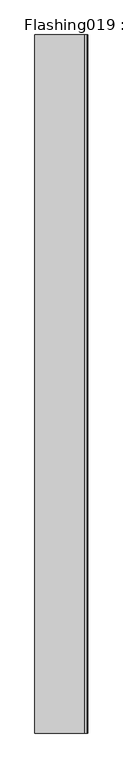
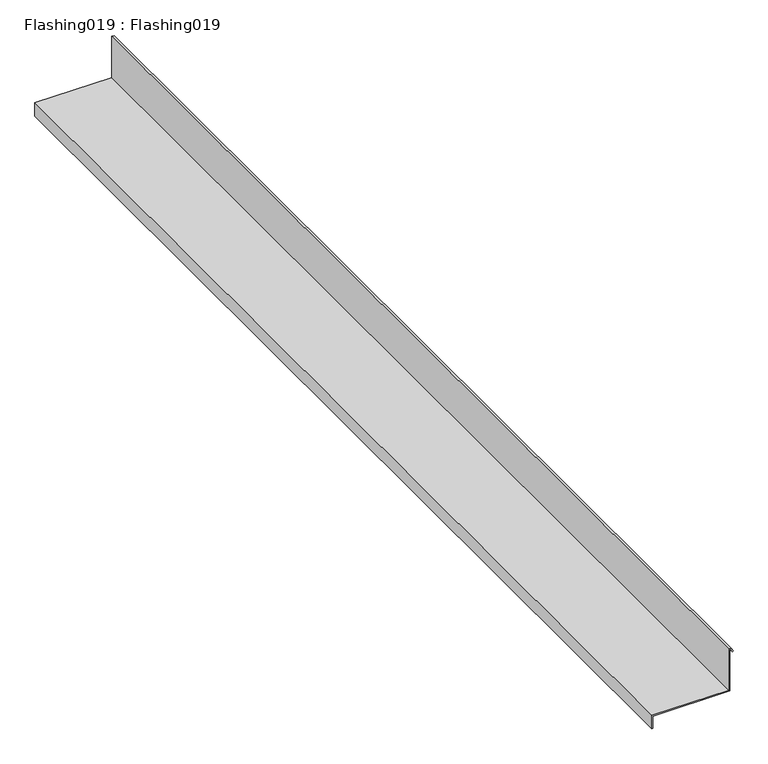
"""IFC4 building model written with IfcOpenShell, lengths in millimetres: proxy geometry, Flashing019 : Flashing019."""

import ifcopenshell
import ifcopenshell.guid

model = None  # the IFC model being written
_history = None  # IfcOwnerHistory: only IFC2X3 demands one
_inside = {}  # id of a spatial element -> (the spatial element, [elements in it])
_under = {}  # id of a project, library or spatial element -> (it, [spatial elements below it])
_declared = {}  # id of a project -> (the project, [libraries it declares])
_typed = {}  # id of a type object -> (the type object, [elements of that type])
_made_of = {}  # id of a material, layer set ... -> (it, [elements and type objects made of it])


def new_model(schema):
    """Start an empty IFC model of exactly this schema.

    Asked for "IFC4X3", IfcOpenShell would pick the latest addendum, in which some entities
    have other attributes; the version numbers below select the first issue.
    IFC2X3 requires an IfcOwnerHistory on every rooted entity: one is made here for all.
    """
    global model, _history
    if schema == "IFC4X3":
        model = ifcopenshell.file(schema_version=(4, 3, 0, 0))
    else:
        model = ifcopenshell.file(schema=schema)
    _inside.clear()
    _under.clear()
    _declared.clear()
    _typed.clear()
    _made_of.clear()
    _history = None
    if model.schema == "IFC2X3":
        org = make("IfcOrganization", Name="unknown")
        user = make(
            "IfcPersonAndOrganization",
            ThePerson=make("IfcPerson", FamilyName="unknown"),
            TheOrganization=org,
        )
        app = make(
            "IfcApplication",
            ApplicationDeveloper=org,
            Version="unknown",
            ApplicationFullName="unknown",
            ApplicationIdentifier="unknown",
        )
        _history = make(
            "IfcOwnerHistory",
            OwningUser=user,
            OwningApplication=app,
            ChangeAction="ADDED",
            CreationDate=0,
        )
    return model


def make(cls, **values):
    """One entity of the class cls with the attributes given. An attribute that is None is left unset."""
    return model.create_entity(
        cls, **{name: value for name, value in values.items() if value is not None}
    )


def rooted(cls, **values):
    """An entity with a GlobalId (a new one), such as an element, a storey or a relation."""
    return make(cls, GlobalId=ifcopenshell.guid.new(), OwnerHistory=_history, **values)


def si_unit(unit_type, name, prefix=None):
    """IfcSIUnit, for example si_unit("LENGTHUNIT", "METRE", prefix="MILLI")."""
    return make("IfcSIUnit", UnitType=unit_type, Prefix=prefix, Name=name)


def assignment(units):
    """IfcUnitAssignment: the units of a project."""
    return None if units is None else make("IfcUnitAssignment", Units=units)


def point(xyz):
    """IfcCartesianPoint."""
    return None if xyz is None else make("IfcCartesianPoint", Coordinates=xyz)


def direction(xyz):
    """IfcDirection."""
    return None if xyz is None else make("IfcDirection", DirectionRatios=xyz)


def frame(location, z_axis=None, x_axis=None):
    """IfcAxis2Placement3D, a coordinate frame: its origin and axes. An axis left out is left unset."""
    return make(
        "IfcAxis2Placement3D",
        Location=point(location),
        Axis=direction(z_axis),
        RefDirection=direction(x_axis),
    )


def origin():
    """The frame at (0, 0, 0) with its axes left unset."""
    return frame((0.0, 0.0, 0.0))


def place(relative_to, where):
    """IfcLocalPlacement: puts the frame where relative to a parent placement (None: the world)."""
    return make(
        "IfcLocalPlacement", PlacementRelTo=relative_to, RelativePlacement=where
    )


def context(
    kind, dimensions, precision=None, world=None, true_north=None, identifier=None
):
    """IfcGeometricRepresentationContext, for example the 3D "Model" context."""
    return make(
        "IfcGeometricRepresentationContext",
        ContextIdentifier=identifier,
        ContextType=kind,
        CoordinateSpaceDimension=dimensions,
        Precision=precision,
        WorldCoordinateSystem=world,
        TrueNorth=true_north,
    )


def project(units=None, contexts=None):
    """IfcProject with its units and contexts."""
    return rooted(
        "IfcProject",
        Name="project",
        RepresentationContexts=contexts,
        UnitsInContext=assignment(units),
    )


def spatial(cls, under=None, at=None, **own):
    """A site, building, storey or space (cls), placed at a placement, below another one or the project."""
    s = rooted(cls, ObjectPlacement=at, **own)
    if under is not None:
        _under.setdefault(under.id(), (under, []))[1].append(s)
    return s


def polyline(points):
    """IfcPolyline through the points."""
    return make("IfcPolyline", Points=[point(p) for p in points])


def outline(outer, holes=None, kind="AREA"):
    """IfcArbitraryClosedProfileDef: a profile drawn as a closed curve; with holes, ...WithVoids."""
    if holes is None:
        return make("IfcArbitraryClosedProfileDef", ProfileType=kind, OuterCurve=outer)
    return make(
        "IfcArbitraryProfileDefWithVoids",
        ProfileType=kind,
        OuterCurve=outer,
        InnerCurves=holes,
    )


def extrude(swept, where, along, depth):
    """IfcExtrudedAreaSolid: the profile swept, set in the frame where, extruded along a direction by depth."""
    return make(
        "IfcExtrudedAreaSolid",
        SweptArea=swept,
        Position=where,
        ExtrudedDirection=direction(along),
        Depth=depth,
    )


def shape(context_of_items, identifier, shape_type, items):
    """IfcShapeRepresentation: the items that make up one representation, for example the "Body"."""
    return make(
        "IfcShapeRepresentation",
        ContextOfItems=context_of_items,
        RepresentationIdentifier=identifier,
        RepresentationType=shape_type,
        Items=items,
    )


def source(mapping_origin, context_of_items, identifier, shape_type, items):
    """IfcRepresentationMap: a shape defined once, which mapped items show again and again."""
    return make(
        "IfcRepresentationMap",
        MappingOrigin=mapping_origin,
        MappedRepresentation=shape(context_of_items, identifier, shape_type, items),
    )


def transform(
    local_origin,
    x_axis=None,
    y_axis=None,
    z_axis=None,
    scale=None,
    scale2=None,
    scale3=None,
    uniform=True,
):
    """IfcCartesianTransformationOperator3D, or its non-uniform kind. x_axis, y_axis, z_axis: its Axis1, 2, 3."""
    if uniform:
        return make(
            "IfcCartesianTransformationOperator3D",
            Axis1=direction(x_axis),
            Axis2=direction(y_axis),
            LocalOrigin=point(local_origin),
            Scale=scale,
            Axis3=direction(z_axis),
        )
    return make(
        "IfcCartesianTransformationOperator3DnonUniform",
        Axis1=direction(x_axis),
        Axis2=direction(y_axis),
        LocalOrigin=point(local_origin),
        Scale=scale,
        Axis3=direction(z_axis),
        Scale2=scale2,
        Scale3=scale3,
    )


def mapped(mapping_source, mapping_target):
    """IfcMappedItem: shows the shape of a source again, moved by a transform."""
    return make(
        "IfcMappedItem", MappingSource=mapping_source, MappingTarget=mapping_target
    )


def made_of(thing, what):
    """Note that an element or type object is made of a material, layer set ...; save() writes the relation."""
    if what is not None:
        _made_of.setdefault(what.id(), (what, []))[1].append(thing)
    return thing


def element(
    cls,
    number,
    at=None,
    inside=None,
    cuts=None,
    type_object=None,
    material=None,
    context=None,
    identifier="Body",
    shape_type=None,
    held_by="IfcProductDefinitionShape",
    body=None,
    shapes=None,
    **own,
):
    """One element of the class cls, such as IfcWall. Its Tag is "e" and its number.

    at: its placement. inside: the storey or other place that contains it. cuts: it is an
    opening in that element (IfcRelVoidsElement). A single representation is given by context,
    identifier, shape_type and body (its items); several are given by shapes. held_by: the class
    of the entity that holds the representations. save() writes the other relations.
    """
    e = rooted(cls, Tag="e%d" % number, ObjectPlacement=at, **own)
    if body is not None:
        shapes = [shape(context, identifier, shape_type, body)]
    if shapes is not None:
        e.Representation = make(held_by, Representations=shapes)
    if inside is not None:
        _inside.setdefault(inside.id(), (inside, []))[1].append(e)
    if cuts is not None:
        rooted(
            "IfcRelVoidsElement", RelatingBuildingElement=cuts, RelatedOpeningElement=e
        )
    if type_object is not None:
        _typed.setdefault(type_object.id(), (type_object, []))[1].append(e)
    return made_of(e, material)


def aggregate(whole, parts):
    """IfcRelAggregates: a whole, such as a stair, and the parts it consists of."""
    return rooted("IfcRelAggregates", RelatingObject=whole, RelatedObjects=parts)


def save(model, path):
    """Write the relations noted so far, then the file.

    IfcRelAggregates (storeys below a building ...), IfcRelContainedInSpatialStructure (elements
    in a storey), IfcRelDefinesByType, IfcRelAssociatesMaterial and IfcRelDeclares: one each for
    every whole, place, type object, material and project.
    """
    for whole, parts in _under.values():
        aggregate(whole, parts)
    for where, things in _inside.values():
        rooted(
            "IfcRelContainedInSpatialStructure",
            RelatedElements=things,
            RelatingStructure=where,
        )
    for kind, things in _typed.values():
        rooted("IfcRelDefinesByType", RelatedObjects=things, RelatingType=kind)
    for what, things in _made_of.values():
        rooted("IfcRelAssociatesMaterial", RelatedObjects=things, RelatingMaterial=what)
    for by, libraries in _declared.values():
        rooted("IfcRelDeclares", RelatingContext=by, RelatedDefinitions=libraries)
    model.write(path)


def flashing019_flashing019_9dc0ec64(model_context):
    return source(origin(), model_context, "Body", "SweptSolid", [
        extrude(outline(polyline([(40784.7382813, 16649.96875), (40784.7382813, 16645.2851562), (40703.2466161, 16645.2851562), (40703.2466161, 16501.84375), (40677.1179688, 16501.84375), (40677.1179688, 16503.84375), (40701.2466161, 16503.84375), (40701.2466161, 16647.2851563), (40782.7382813, 16647.2851563), (40782.7382813, 16648.7903893), (40776.8666698, 16652.0435345), (40777.8359375, 16653.7929687), (40784.7382813, 16649.96875)])), frame((0.0, 7982.1449366, 0.0), z_axis=(0.0, 1.0, 0.0), x_axis=(0.0, 0.0, 1.0)), (0.0, 0.0, 1.0), 2000.0),
    ])


if __name__ == "__main__":
    model = new_model("IFC4")
    model_context = context("Model", 3, world=origin())
    ifc_project = project(units=[si_unit("LENGTHUNIT", "METRE", prefix="MILLI")], contexts=[model_context])
    site = spatial("IfcSite", under=ifc_project)
    building = spatial("IfcBuilding", under=site)
    placement = place(None, origin())
    flashing019_flashing019_shape = flashing019_flashing019_9dc0ec64(model_context)
    element("IfcBuildingElementProxy", 1, Name="Flashing019 : Flashing019", ObjectType="Flashing019 : Flashing019", at=placement, inside=building, context=model_context, shape_type="MappedRepresentation", body=[
        mapped(flashing019_flashing019_shape, transform((0.0, 0.0, 0.0), x_axis=(1.0, 0.0, 0.0), y_axis=(0.0, 1.0, 0.0), z_axis=(0.0, 0.0, 1.0))),
    ])
    save(model, "model.ifc")

# Revit data of these elements
# Type "Flashing019 : Flashing019"
#   NameOverride = "Flashing019"
# Element 1 (IfcBuildingElementProxy, "Flashing019 : Flashing019")
#   Materials on its faces: "BRAKE METAL TO WRAP FRAMING OVER BITUTHANE"
# Materials
#   "BRAKE METAL TO WRAP FRAMING OVER BITUTHANE": class "Unassigned", colour RGB 128 128 128, transparency 0, Cost = 0
